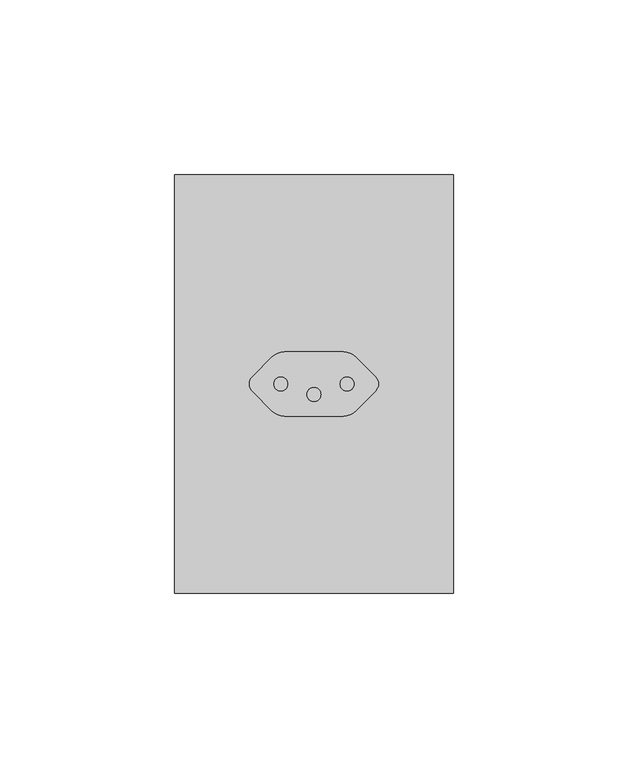
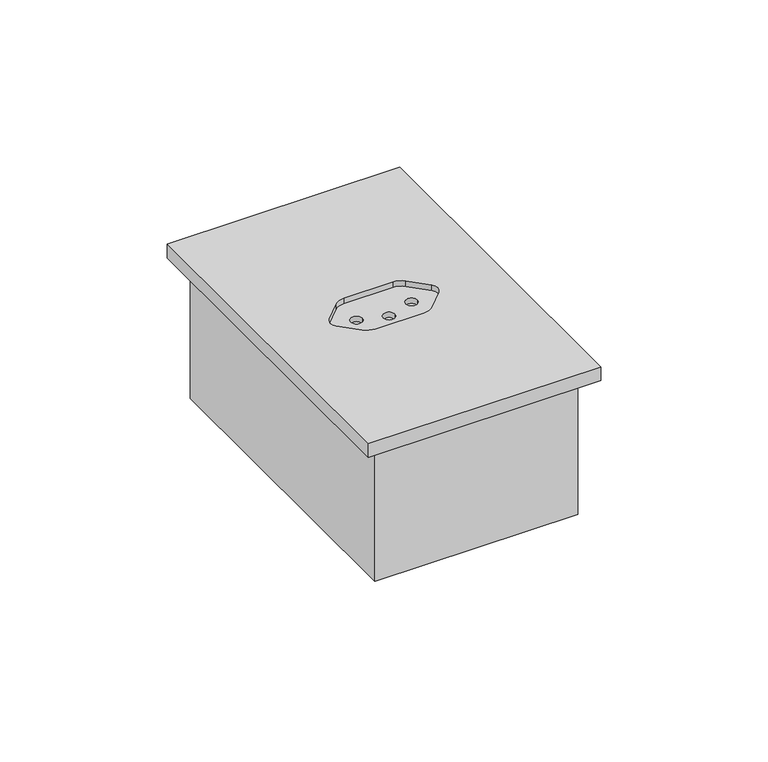
"""IFC4 building model written with IfcOpenShell, lengths in millimetres: proxy geometry, CAIXA VERTICE V7 : Tomada 10A 1s."""

from ifc_helpers import new_model, si_unit, frame, origin, place, context, project, spatial, polyline, circle_curve, faceted_brep, source, transform, mapped, element, save
from ifc_brep_helpers import plane_surface, revolved_surface, advanced_brep


def electrical_fixtures_a0445b9b(model_context):
    return source(origin(), model_context, "Body", "SolidModel", [
        faceted_brep([(35.0, -1155.0, 0.0), (35.0, -1045.0, 0.0), (-35.0, -1045.0, 0.0), (-35.0, -1155.0, 0.0), (33.0, -1153.0, 0.0), (-33.0, -1153.0, 0.0), (-33.0, -1047.0, 0.0), (33.0, -1047.0, 0.0), (33.0, -1047.0, -48.0), (-33.0, -1047.0, -48.0), (-33.0, -1153.0, -48.0), (33.0, -1153.0, -48.0), (35.0, -1155.0, -50.0), (-35.0, -1155.0, -50.0), (-35.0, -1045.0, -50.0), (35.0, -1045.0, -50.0)], [[[0, 1, 2, 3], [4, 5, 6, 7]], [[8, 9, 10, 11]], [[12, 13, 14, 15]], [[12, 0, 3, 13]], [[3, 2, 14, 13]], [[2, 1, 15, 14]], [[1, 0, 12, 15]], [[7, 8, 11, 4]], [[6, 9, 8, 7]], [[5, 10, 9, 6]], [[4, 11, 10, 5]]]),
        advanced_brep(
        [(40.0, -1160.0, 5.0), (40.0, -1040.0, 5.0), (-40.0, -1040.0, 5.0), (-40.0, -1160.0, 5.0), (8.4215729, -1090.75, 5.0), (11.9571068, -1092.2144661, 5.0), (17.6213203, -1097.8786797, 5.0), (17.6213203, -1102.1213203, 5.0), (11.9571068, -1107.7855339, 5.0), (8.4215729, -1109.25, 5.0), (-8.4215729, -1109.25, 5.0), (-11.9571068, -1107.7855339, 5.0), (-17.6213203, -1102.1213203, 5.0), (-17.6213203, -1097.8786797, 5.0), (-11.9571068, -1092.2144661, 5.0), (-8.4215729, -1090.75, 5.0), (-40.0, -1160.0, 0.0), (-40.0, -1040.0, 0.0), (40.0, -1040.0, 0.0), (40.0, -1160.0, 0.0), (8.4215729, -1090.75, 3.0), (-8.4215729, -1090.75, 3.0), (-11.9571068, -1092.2144661, 3.0), (-17.6213203, -1097.8786797, 3.0), (-17.6213203, -1102.1213203, 3.0), (-11.9571068, -1107.7855339, 3.0), (-8.4215729, -1109.25, 3.0), (8.4215729, -1109.25, 3.0), (11.9571068, -1107.7855339, 3.0), (17.6213203, -1102.1213203, 3.0), (17.6213203, -1097.8786797, 3.0), (11.9571068, -1092.2144661, 3.0), (-7.5, -1100.0, 3.0), (-11.5, -1100.0, 3.0), (11.5, -1100.0, 3.0), (7.5, -1100.0, 3.0), (2.0, -1103.0, 3.0), (-2.0, -1103.0, 3.0), (-11.5, -1100.0, 1.0), (-7.5, -1100.0, 1.0), (7.5, -1100.0, 1.0), (11.5, -1100.0, 1.0), (-2.0, -1103.0, 1.0), (2.0, -1103.0, 1.0)],
        [
            (0, 1),
            (1, 2),
            (2, 3),
            (3, 0),
            (4, 5, circle_curve(frame((8.4215729, -1095.75, 5.0), z_axis=(0.0, 0.0, -1.0), x_axis=(-1.0, 0.0, 0.0)), 5.0)),
            (5, 6),
            (6, 7, circle_curve(frame((15.5, -1100.0, 5.0), z_axis=(0.0, 0.0, -1.0), x_axis=(-1.0, 0.0, 0.0)), 3.0)),
            (7, 8),
            (8, 9, circle_curve(frame((8.4215729, -1104.25, 5.0), z_axis=(0.0, 0.0, -1.0), x_axis=(-1.0, 0.0, 0.0)), 5.0)),
            (9, 10),
            (10, 11, circle_curve(frame((-8.4215729, -1104.25, 5.0), z_axis=(0.0, 0.0, -1.0), x_axis=(-1.0, 0.0, 0.0)), 5.0)),
            (11, 12),
            (12, 13, circle_curve(frame((-15.5, -1100.0, 5.0), z_axis=(0.0, 0.0, -1.0), x_axis=(-1.0, 0.0, 0.0)), 3.0)),
            (13, 14),
            (14, 15, circle_curve(frame((-8.4215729, -1095.75, 5.0), z_axis=(0.0, 0.0, -1.0), x_axis=(-1.0, 0.0, 0.0)), 5.0)),
            (15, 4),
            (16, 17),
            (17, 18),
            (18, 19),
            (19, 16),
            (3, 16),
            (19, 0),
            (2, 17),
            (1, 18),
            (20, 21),
            (21, 22, circle_curve(frame((-8.4215729, -1095.75, 3.0), z_axis=(0.0, 0.0, 1.0), x_axis=(-1.0, 0.0, 0.0)), 5.0)),
            (22, 23),
            (23, 24, circle_curve(frame((-15.5, -1100.0, 3.0), z_axis=(0.0, 0.0, 1.0), x_axis=(-1.0, 0.0, 0.0)), 3.0)),
            (24, 25),
            (25, 26, circle_curve(frame((-8.4215729, -1104.25, 3.0), z_axis=(0.0, 0.0, 1.0), x_axis=(-1.0, 0.0, 0.0)), 5.0)),
            (26, 27),
            (27, 28, circle_curve(frame((8.4215729, -1104.25, 3.0), z_axis=(0.0, 0.0, 1.0), x_axis=(-1.0, 0.0, 0.0)), 5.0)),
            (28, 29),
            (29, 30, circle_curve(frame((15.5, -1100.0, 3.0), z_axis=(0.0, 0.0, 1.0), x_axis=(-1.0, 0.0, 0.0)), 3.0)),
            (30, 31),
            (31, 20, circle_curve(frame((8.4215729, -1095.75, 3.0), z_axis=(0.0, 0.0, 1.0), x_axis=(-1.0, 0.0, 0.0)), 5.0)),
            (32, 33, circle_curve(frame((-9.5, -1100.0, 3.0), z_axis=(0.0, 0.0, -1.0), x_axis=(1.0, -2.301812013077709e-12, 0.0)), 2.0)),
            (33, 32, circle_curve(frame((-9.5, -1100.0, 3.0), z_axis=(0.0, 0.0, -1.0), x_axis=(1.0, -2.301812013077709e-12, 0.0)), 2.0)),
            (34, 35, circle_curve(frame((9.5, -1100.0, 3.0), z_axis=(0.0, 0.0, -1.0), x_axis=(1.0, -2.301812013077709e-12, 0.0)), 2.0)),
            (35, 34, circle_curve(frame((9.5, -1100.0, 3.0), z_axis=(0.0, 0.0, -1.0), x_axis=(1.0, -2.301812013077709e-12, 0.0)), 2.0)),
            (36, 37, circle_curve(frame((0.0, -1103.0, 3.0), z_axis=(0.0, 0.0, -1.0), x_axis=(1.0, -2.301812013077709e-12, 0.0)), 2.0)),
            (37, 36, circle_curve(frame((0.0, -1103.0, 3.0), z_axis=(0.0, 0.0, -1.0), x_axis=(1.0, -2.301812013077709e-12, 0.0)), 2.0)),
            (20, 4),
            (15, 21),
            (14, 22),
            (13, 23),
            (12, 24),
            (11, 25),
            (10, 26),
            (9, 27),
            (8, 28),
            (7, 29),
            (6, 30),
            (5, 31),
            (38, 39, circle_curve(frame((-9.5, -1100.0, 1.0), z_axis=(0.0, 0.0, 1.0), x_axis=(1.0, -2.301812013077709e-12, 0.0)), 2.0)),
            (39, 38, circle_curve(frame((-9.5, -1100.0, 1.0), z_axis=(0.0, 0.0, 1.0), x_axis=(1.0, -2.301812013077709e-12, 0.0)), 2.0)),
            (40, 41, circle_curve(frame((9.5, -1100.0, 1.0), z_axis=(0.0, 0.0, 1.0), x_axis=(1.0, -2.301812013077709e-12, 0.0)), 2.0)),
            (41, 40, circle_curve(frame((9.5, -1100.0, 1.0), z_axis=(0.0, 0.0, 1.0), x_axis=(1.0, -2.301812013077709e-12, 0.0)), 2.0)),
            (42, 43, circle_curve(frame((0.0, -1103.0, 1.0), z_axis=(0.0, 0.0, 1.0), x_axis=(1.0, -2.301812013077709e-12, 0.0)), 2.0)),
            (43, 42, circle_curve(frame((0.0, -1103.0, 1.0), z_axis=(0.0, 0.0, 1.0), x_axis=(1.0, -2.301812013077709e-12, 0.0)), 2.0)),
            (33, 38),
            (39, 32),
            (35, 40),
            (41, 34),
            (37, 42),
            (43, 36),
        ],
        [
            plane_surface(frame((-60.0, -1160.0, 5.0), z_axis=(0.0, 0.0, 1.0), x_axis=(-1.0, 0.0, 0.0))),
            plane_surface(frame((-60.0, -1160.0, 0.0), z_axis=(0.0, 0.0, -1.0), x_axis=(1.0, 0.0, 0.0))),
            plane_surface(frame((40.0, -1160.0, 5.0), z_axis=(0.0, -1.0, 0.0), x_axis=(0.0, 0.0, -1.0))),
            plane_surface(frame((-40.0, -1160.0, 5.0), z_axis=(-1.0, 0.0, 0.0), x_axis=(0.0, 0.0, -1.0))),
            plane_surface(frame((-40.0, -1040.0, 5.0), z_axis=(0.0, 1.0, 0.0), x_axis=(0.0, 0.0, -1.0))),
            plane_surface(frame((40.0, -1040.0, 5.0), z_axis=(1.0, 0.0, 0.0), x_axis=(0.0, 0.0, -1.0))),
            plane_surface(frame((3.4215729, -1095.75, 3.0), z_axis=(0.0, 0.0, 1.0), x_axis=(0.0, -1.0, 0.0))),
            plane_surface(frame((-8.4215729, -1090.75, 5.0), z_axis=(0.0, -1.0, 0.0), x_axis=(0.0, 0.0, -1.0))),
            revolved_surface(polyline([(-13.4215729, -1095.75, 5.0), (-13.4215729, -1095.75, 3.0)]), (-8.4215729, -1095.75, 3.0), (0.0, 0.0, 1.0)),
            plane_surface(frame((-17.6213203, -1097.8786797, 5.0), z_axis=(0.7071067811865045, -0.7071067811865905, 0.0), x_axis=(0.0, 0.0, -1.0))),
            revolved_surface(polyline([(-18.5, -1100.0, 5.0), (-18.5, -1100.0, 3.0)]), (-15.5, -1100.0, 3.0), (0.0, 0.0, 1.0)),
            plane_surface(frame((-11.9571068, -1107.7855339, 5.0), z_axis=(0.7071067811865515, 0.7071067811865437, 0.0), x_axis=(0.0, 0.0, -1.0))),
            revolved_surface(polyline([(-13.4215729, -1104.25, 5.0), (-13.4215729, -1104.25, 3.0)]), (-8.4215729, -1104.25, 3.0), (0.0, 0.0, 1.0)),
            plane_surface(frame((8.4215729, -1109.25, 5.0), z_axis=(0.0, 1.0, 0.0), x_axis=(0.0, 0.0, -1.0))),
            revolved_surface(polyline([(3.4215728999999993, -1104.25, 5.0), (3.4215728999999993, -1104.25, 3.0)]), (8.4215729, -1104.25, 3.0), (0.0, 0.0, 1.0)),
            plane_surface(frame((17.6213203, -1102.1213203, 5.0), z_axis=(-0.7071067811865307, 0.7071067811865643, 0.0), x_axis=(0.0, 0.0, -1.0))),
            revolved_surface(polyline([(12.5, -1100.0, 5.0), (12.5, -1100.0, 3.0)]), (15.5, -1100.0, 3.0), (0.0, 0.0, 1.0)),
            plane_surface(frame((11.9571068, -1092.2144661, 5.0), z_axis=(-0.7071067811865893, -0.7071067811865058, 0.0), x_axis=(0.0, 0.0, -1.0))),
            revolved_surface(polyline([(3.4215728999999993, -1095.75, 5.0), (3.4215728999999993, -1095.75, 3.0)]), (8.4215729, -1095.75, 3.0), (0.0, 0.0, 1.0)),
            plane_surface(frame((-7.5, -1100.0, 1.0), z_axis=(0.0, 0.0, 1.0), x_axis=(2.301812013077709e-12, 1.0, 0.0))),
            revolved_surface(polyline([(-7.5, -1100.0000000000045, 3.0), (-7.5, -1100.0000000000045, 1.0)]), (-9.5, -1100.0, 1.0), (0.0, 0.0, 1.0)),
            revolved_surface(polyline([(11.5, -1100.0000000000045, 3.0), (11.5, -1100.0000000000045, 1.0)]), (9.5, -1100.0, 5.0), (0.0, 0.0, 1.0)),
            revolved_surface(polyline([(2.0, -1103.0000000000045, 3.0), (2.0, -1103.0000000000045, 1.0)]), (0.0, -1103.0, 5.0), (0.0, 0.0, 1.0)),
        ],
        [
            (0, [[1, 2, 3, 4], [5, 6, 7, 8, 9, 10, 11, 12, 13, 14, 15, 16]]),
            (1, [[17, 18, 19, 20]]),
            (2, [[21, -20, 22, -4]]),
            (3, [[23, -17, -21, -3]]),
            (4, [[24, -18, -23, -2]]),
            (5, [[-22, -19, -24, -1]]),
            (6, [[25, 26, 27, 28, 29, 30, 31, 32, 33, 34, 35, 36], [37, 38], [39, 40], [41, 42]]),
            (7, [[43, -16, 44, -25]]),
            (8, [[-44, -15, 45, -26]]),
            (9, [[-45, -14, 46, -27]]),
            (10, [[-46, -13, 47, -28]]),
            (11, [[-47, -12, 48, -29]]),
            (12, [[-48, -11, 49, -30]]),
            (13, [[-49, -10, 50, -31]]),
            (14, [[-50, -9, 51, -32]]),
            (15, [[-51, -8, 52, -33]]),
            (16, [[-52, -7, 53, -34]]),
            (17, [[-53, -6, 54, -35]]),
            (18, [[-54, -5, -43, -36]]),
            (19, [[55, 56]]),
            (19, [[57, 58]]),
            (19, [[59, 60]]),
            (20, [[61, -56, 62, -38]]),
            (20, [[-62, -55, -61, -37]]),
            (21, [[63, -58, 64, -40]]),
            (21, [[-64, -57, -63, -39]]),
            (22, [[65, -60, 66, -42]]),
            (22, [[-66, -59, -65, -41]]),
        ],
    ),
    ])


if __name__ == "__main__":
    model = new_model("IFC4")
    model_context = context("Model", 3, world=origin())
    ifc_project = project(units=[si_unit("LENGTHUNIT", "METRE", prefix="MILLI")], contexts=[model_context])
    site = spatial("IfcSite", under=ifc_project)
    building = spatial("IfcBuilding", under=site)
    placement = place(None, origin())
    electrical_fixtures_shape = electrical_fixtures_a0445b9b(model_context)
    element("IfcBuildingElementProxy", 1, Name="CAIXA VERTICE V7 : Tomada 10A 1s", ObjectType="CAIXA VERTICE V7 : Tomada 10A 1s", at=placement, inside=building, context=model_context, shape_type="MappedRepresentation", body=[
        mapped(electrical_fixtures_shape, transform((0.0, 0.0, 0.0), x_axis=(1.0, 0.0, 0.0), y_axis=(0.0, 1.0, 0.0), z_axis=(0.0, 0.0, 1.0))),
    ])
    save(model, "model.ifc")

# Revit data of these elements
# Type "CAIXA VERTICE V7 : Tomada 10A 1s"
#   URL = "www.facebook.com/verticetreinamentos"
#   SEÇÃO [instance default] = ""
#   Rotação [instance default] = 0.00°
#   LARGURA DA TAMPA = 0.08 m
#   BORDA = 0.01 m
#   ALTURA DE INSTALAÇÃO [instance default] = 1.10 m
#   Distância Anotação [instance default] = 0.0015 m
#   ALTURA DA TAMPA = 0.12 m
#   Vertical [instance default] = yes
#   VER SEÇÃO [instance default] = no
#   SHADE ESQ [instance default] = no
#   SHADE DIR [instance default] = yes
#   HORIZONTAL [instance default] = no
#   ANDAR COM A LEGENDA [instance default] = 0
#   Material Tampa [instance default] = Plástico, branco opaco
#   Caixa = element 1798514
#   Anotação = element 1798528
#   Default Elevation = 0
# Element 1 (IfcBuildingElementProxy, "CAIXA VERTICE V7 : Tomada 10A 1s")
#   Materials on its faces: "Plástico, branco opaco"
# Materials
#   "Plástico, branco opaco": class "Plástico", colour RGB 120 120 120, transparency 0, Description = "Plastic, generic, opaque white", Cost = 0
